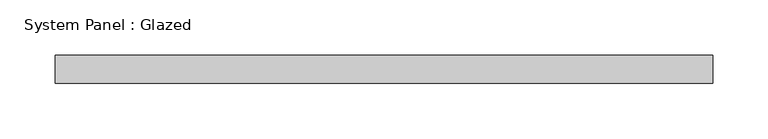
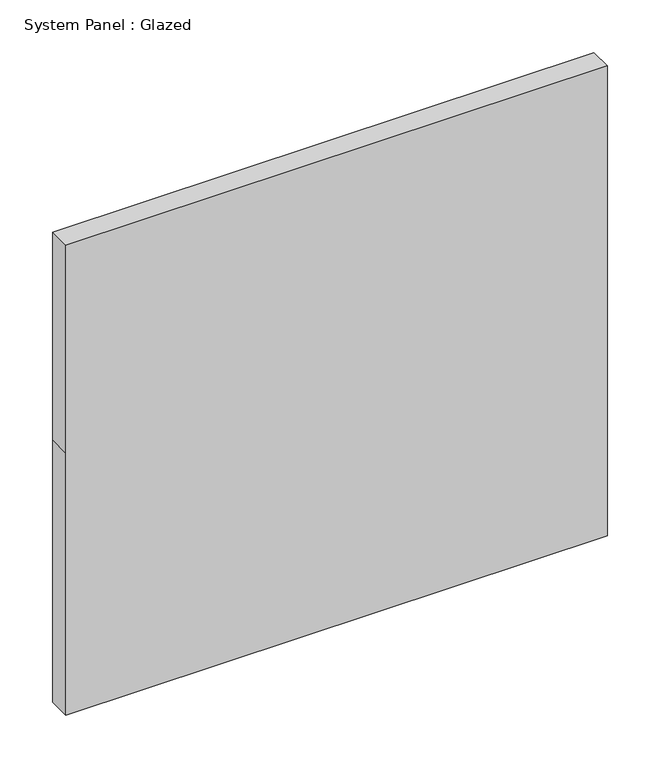
"""IFC4 building model written with IfcOpenShell, lengths in millimetres: plate geometry, System Panel : Glazed."""

from ifc_helpers import new_model, si_unit, frame, origin, place, context, project, spatial, polyline, outline, extrude, source, transform, mapped, element, save


def system_panel_glazed_65392b54(model_context):
    return source(origin(), model_context, "Body", "SweptSolid", [
        extrude(outline(polyline([(0.0, -297.7), (0.0, 297.7), (304.8, 297.7), (546.1, 297.7), (546.1, -297.7), (304.8, -297.7), (0.0, -297.7)])), frame((0.0, -44.45, 0.0), z_axis=(0.0, 1.0, 0.0), x_axis=(0.0, 0.0, 1.0)), (0.0, 0.0, 1.0), 25.4),
    ])


if __name__ == "__main__":
    model = new_model("IFC4")
    model_context = context("Model", 3, world=origin())
    ifc_project = project(units=[si_unit("LENGTHUNIT", "METRE", prefix="MILLI")], contexts=[model_context])
    site = spatial("IfcSite", under=ifc_project)
    building = spatial("IfcBuilding", under=site)
    placement = place(None, origin())
    system_panel_glazed_shape = system_panel_glazed_65392b54(model_context)
    element("IfcPlate", 1, ObjectType="System Panel : Glazed", at=placement, inside=building, context=model_context, shape_type="MappedRepresentation", body=[
        mapped(system_panel_glazed_shape, transform((0.0, 0.0, 0.0), x_axis=(1.0, 0.0, 0.0), y_axis=(0.0, 1.0, 0.0), z_axis=(0.0, 0.0, 1.0))),
    ])
    save(model, "model.ifc")

# Revit data of these elements
# Element 1 (IfcPlate, "System Panel : Glazed")
#   Materials on its faces: "Glass"
# Materials
#   "Glass": class "Glass", colour RGB 0 128 192, transparency 0.75
